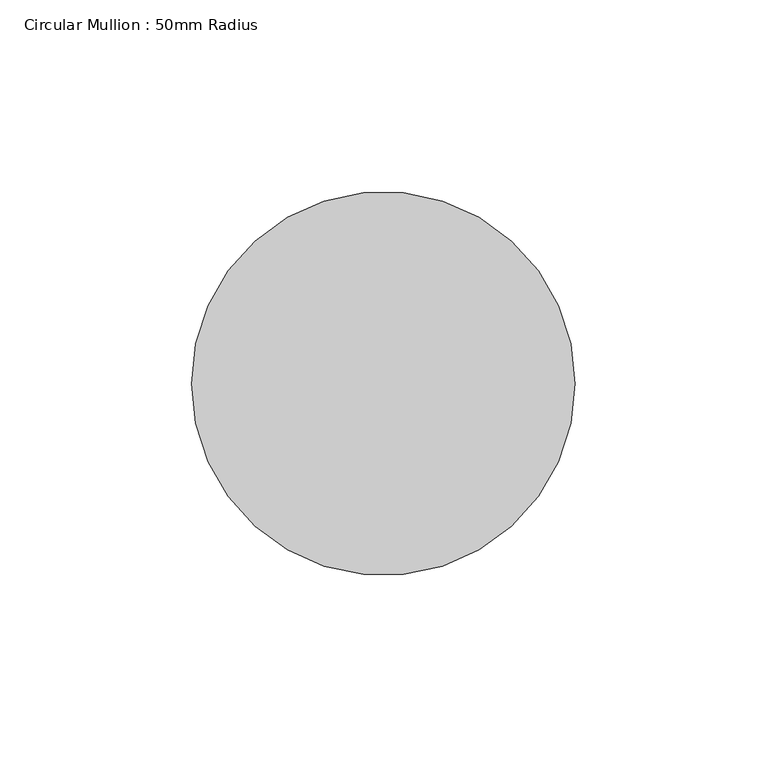
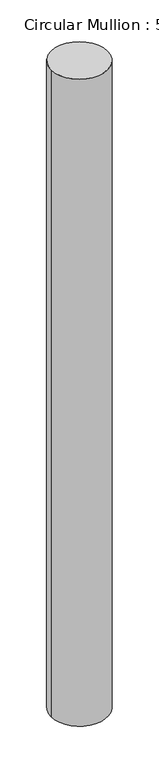
"""IFC4 building model written with IfcOpenShell, lengths in millimetres: member geometry, Circular Mullion : 50mm Radius."""

from ifc_helpers import new_model, si_unit, point, frame, origin, origin_2d, place, context, project, spatial, circle_curve, trimmed, segment, composite_curve, outline, extrude, source, transform, mapped, element, save


def circular_mullion_50mm_radius_f12a6cae(model_context):
    return source(origin(), model_context, "Body", "SweptSolid", [
        extrude(outline(composite_curve([segment(trimmed(circle_curve(origin_2d(), 50.0), [point((50.0, 0.0))], [point((-50.0, 0.0))], False, "CARTESIAN"), True, "CONTINUOUS"), segment(trimmed(circle_curve(origin_2d(), 50.0), [point((-50.0, 0.0))], [point((50.0, 0.0))], False, "CARTESIAN"), True, "CONTINUOUS")], self_intersect=False)), frame((0.0, 0.0, -1208.1443654), z_axis=(0.0, 0.0, 1.0), x_axis=(1.0, 0.0, 0.0)), (0.0, 0.0, 1.0), 1208.1443654),
    ])


if __name__ == "__main__":
    model = new_model("IFC4")
    model_context = context("Model", 3, world=origin())
    ifc_project = project(units=[si_unit("LENGTHUNIT", "METRE", prefix="MILLI")], contexts=[model_context])
    site = spatial("IfcSite", under=ifc_project)
    building = spatial("IfcBuilding", under=site)
    placement = place(None, origin())
    circular_mullion_50mm_radius_shape = circular_mullion_50mm_radius_f12a6cae(model_context)
    element("IfcMember", 1, ObjectType="Circular Mullion : 50mm Radius", at=placement, inside=building, context=model_context, shape_type="MappedRepresentation", body=[
        mapped(circular_mullion_50mm_radius_shape, transform((0.0, 0.0, 0.0), x_axis=(1.0, 0.0, 0.0), y_axis=(0.0, 1.0, 0.0), z_axis=(0.0, 0.0, 1.0))),
    ])
    save(model, "model.ifc")

# Revit data of these elements
# Type "Circular Mullion : 50mm Radius"
#   built-in parameter 1007350 = 0.164042 (stored number, unit not read)
# Element 1 (IfcMember, "Circular Mullion : 50mm Radius")
#   Materials on its faces: "Aluminium"
# Materials
#   "Aluminium": class "Metal", colour RGB 247 247 247, transparency 0, Description = "Aluminium 6061", Cost = 0
